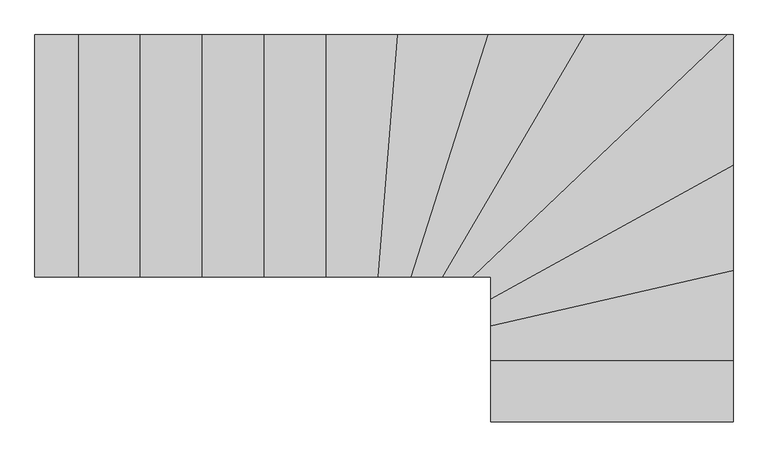
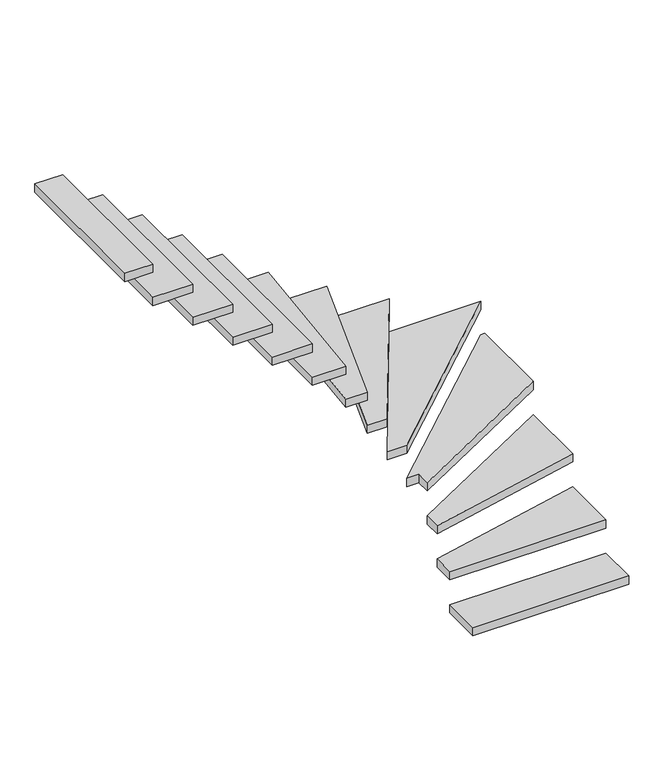
"""IFC4 building model written with IfcOpenShell, lengths in millimetres: stair geometry,   151686 :   151686."""

from ifc_helpers import new_model, si_unit, frame, origin, place, context, project, spatial, polyline, outline, extrude, source, transform, mapped, element, save


def stair_6893023c(model_context):
    return source(origin(), model_context, "Body", "SweptSolid", [
        extrude(outline(polyline([(171517.7593015, 39074.7962965), (172417.7593015, 39074.7962965), (172417.7593015, 38844.7962965), (171517.7593015, 38844.7962965), (171517.7593015, 39074.7962965)])), frame((0.0, 0.0, 3482.1428571), z_axis=(0.0, 0.0, 1.0), x_axis=(1.0, 0.0, 0.0)), (0.0, 0.0, 1.0), 50.0),
        extrude(outline(polyline([(171517.7593015, 39201.8291061), (172417.7593015, 39407.7634868), (172417.7593015, 39074.7962965), (171517.7593015, 39074.7962965), (171517.7593015, 39201.8291061)])), frame((0.0, 0.0, 3684.2857143), z_axis=(0.0, 0.0, 1.0), x_axis=(1.0, 0.0, 0.0)), (0.0, 0.0, 1.0), 50.0),
        extrude(outline(polyline([(171517.7593015, 39301.7193734), (172417.7593015, 39801.0914939), (172417.7593015, 39407.7634868), (171517.7593015, 39201.8291061), (171517.7593015, 39301.7193734)])), frame((0.0, 0.0, 3886.4285714), z_axis=(0.0, 0.0, 1.0), x_axis=(1.0, 0.0, 0.0)), (0.0, 0.0, 1.0), 50.0),
        extrude(outline(polyline([(171517.7593015, 39384.7962965), (171447.7593015, 39384.7962965), (172395.0888853, 40284.7962965), (172417.7593015, 40284.7962965), (172417.7593015, 39801.0914939), (171517.7593015, 39301.7193734), (171517.7593015, 39384.7962965)])), frame((0.0, 0.0, 4088.5714286), z_axis=(0.0, 0.0, 1.0), x_axis=(1.0, 0.0, 0.0)), (0.0, 0.0, 1.0), 50.0),
        extrude(outline(polyline([(171336.7472141, 39384.7962965), (171865.3205791, 40284.7962965), (172395.0888853, 40284.7962965), (171447.7593015, 39384.7962965), (171336.7472141, 39384.7962965)])), frame((0.0, 0.0, 4290.7142857), z_axis=(0.0, 0.0, 1.0), x_axis=(1.0, 0.0, 0.0)), (0.0, 0.0, 1.0), 50.0),
        extrude(outline(polyline([(171220.2248249, 39384.7962965), (171506.0901048, 40284.7962965), (171865.3205791, 40284.7962965), (171336.7472141, 39384.7962965), (171220.2248249, 39384.7962965)])), frame((0.0, 0.0, 4492.8571429), z_axis=(0.0, 0.0, 1.0), x_axis=(1.0, 0.0, 0.0)), (0.0, 0.0, 1.0), 50.0),
        extrude(outline(polyline([(171096.414661, 39384.7962965), (171169.9002687, 40284.7962965), (171506.0901048, 40284.7962965), (171220.2248249, 39384.7962965), (171096.414661, 39384.7962965)])), frame((0.0, 0.0, 4695.0), z_axis=(0.0, 0.0, 1.0), x_axis=(1.0, 0.0, 0.0)), (0.0, 0.0, 1.0), 50.0),
        extrude(outline(polyline([(170903.1574649, 39384.7962965), (170903.1574649, 40284.7962965), (171169.9002687, 40284.7962965), (171096.414661, 39384.7962965), (170903.1574649, 39384.7962965)])), frame((0.0, 0.0, 4897.1428571), z_axis=(0.0, 0.0, 1.0), x_axis=(1.0, 0.0, 0.0)), (0.0, 0.0, 1.0), 50.0),
        extrude(outline(polyline([(170673.1574649, 39384.7962965), (170673.1574649, 40284.7962965), (170903.1574649, 40284.7962965), (170903.1574649, 39384.7962965), (170673.1574649, 39384.7962965)])), frame((0.0, 0.0, 5099.2857143), z_axis=(0.0, 0.0, 1.0), x_axis=(1.0, 0.0, 0.0)), (0.0, 0.0, 1.0), 50.0),
        extrude(outline(polyline([(170443.1574649, 39384.7962965), (170443.1574649, 40284.7962965), (170673.1574649, 40284.7962965), (170673.1574649, 39384.7962965), (170443.1574649, 39384.7962965)])), frame((0.0, 0.0, 5301.4285714), z_axis=(0.0, 0.0, 1.0), x_axis=(1.0, 0.0, 0.0)), (0.0, 0.0, 1.0), 50.0),
        extrude(outline(polyline([(170213.1574649, 39384.7962965), (170213.1574649, 40284.7962965), (170443.1574649, 40284.7962965), (170443.1574649, 39384.7962965), (170213.1574649, 39384.7962965)])), frame((0.0, 0.0, 5503.5714286), z_axis=(0.0, 0.0, 1.0), x_axis=(1.0, 0.0, 0.0)), (0.0, 0.0, 1.0), 50.0),
        extrude(outline(polyline([(169983.1574649, 39384.7962965), (169983.1574649, 40284.7962965), (170213.1574649, 40284.7962965), (170213.1574649, 39384.7962965), (169983.1574649, 39384.7962965)])), frame((0.0, 0.0, 5705.7142857), z_axis=(0.0, 0.0, 1.0), x_axis=(1.0, 0.0, 0.0)), (0.0, 0.0, 1.0), 50.0),
        extrude(outline(polyline([(169822.7593015, 39384.7962965), (169822.7593015, 40284.7962965), (169983.1574649, 40284.7962965), (169983.1574649, 39384.7962965), (169822.7593015, 39384.7962965)])), frame((0.0, 0.0, 5907.8571429), z_axis=(0.0, 0.0, 1.0), x_axis=(1.0, 0.0, 0.0)), (0.0, 0.0, 1.0), 50.0),
    ])


if __name__ == "__main__":
    model = new_model("IFC4")
    model_context = context("Model", 3, world=origin())
    ifc_project = project(units=[si_unit("LENGTHUNIT", "METRE", prefix="MILLI")], contexts=[model_context])
    site = spatial("IfcSite", under=ifc_project)
    building = spatial("IfcBuilding", under=site)
    placement = place(None, origin())
    stair_shape = stair_6893023c(model_context)
    element("IfcStair", 1, ObjectType="  151686 :   151686", at=placement, inside=building, context=model_context, shape_type="MappedRepresentation", body=[
        mapped(stair_shape, transform((0.0, 0.0, 0.0), x_axis=(1.0, 0.0, 0.0), y_axis=(0.0, 1.0, 0.0), z_axis=(0.0, 0.0, 1.0))),
    ])
    save(model, "model.ifc")

# Revit data of these elements
# Type "  151686 :   151686"
#   Abrechnungsart = "St"
#   Allright_Bauteil_ID = "0131Tre0659044570"
#   Material = "Stahlbeton"
#   Objektname = "Treppe"
#   NameOverride = " "
#   ThermalTransmittance = 0.0000 BTU/(h·ft²·°F)
#   NosingLength = 0.000 m
#   NumberOfRiser = 14
#   NumberOfTreads = 13
#   RiserHeight = 2.021 m
#   TreadLength = 2.300 m
#   IsExternal = no
#   FireExit = no
#   HandicapAccessible = no
#   HasNonSkidSurface = no
# Element 1 (IfcStair, "  151686 :   151686")
#   Materials on its faces: "weiss"
# Materials
#   "weiss": class "Unassigned", colour RGB 255 255 255, transparency 0
